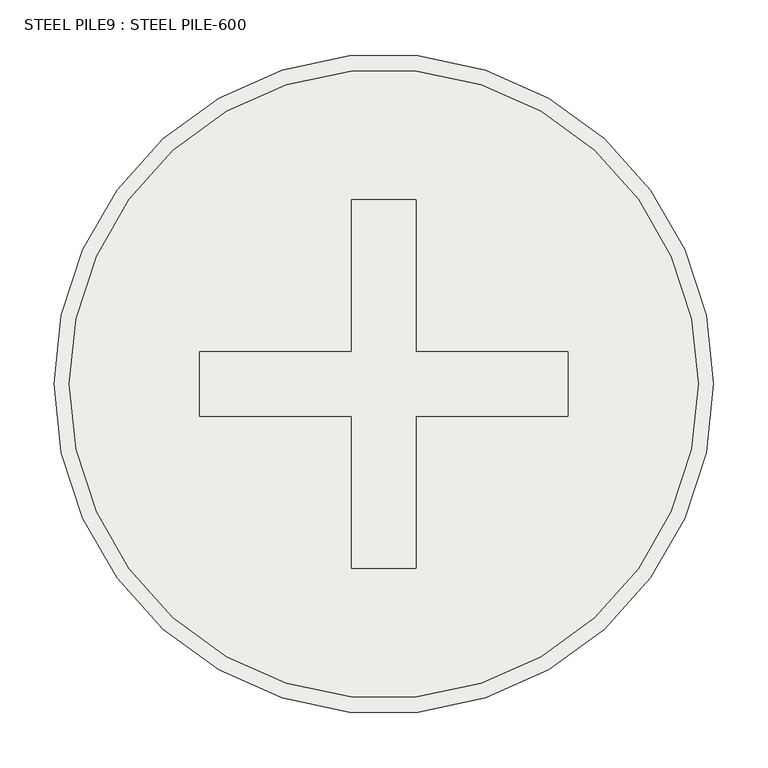
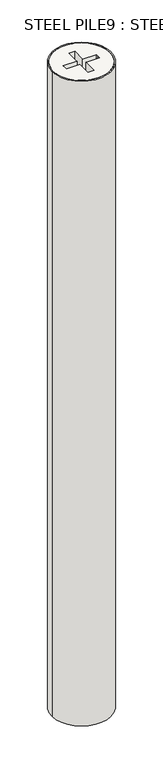
"""IFC4 building model written with IfcOpenShell, lengths in millimetres: slab geometry, STEEL PILE9 : STEEL PILE-600."""

from ifc_helpers import new_model, si_unit, point, frame, frame_2d, origin, place, context, project, spatial, circle_curve, trimmed, segment, composite_curve, outline, extrude, source, transform, mapped, element, save
from ifc_brep_helpers import plane_surface, cylinder_surface, advanced_brep


def steel_pile9_steel_pile_600_482db376(model_context):
    return source(origin(), model_context, "Body", "SolidModel", [
        advanced_brep(
        [(5709.5, 19499.5208589, 150.0), (6290.5, 19499.5208589, 150.0), (5970.0, 19469.5208589, 150.0), (5830.0, 19469.5208589, 150.0), (5830.0, 19499.5208589, 150.0), (5830.0, 19529.5208589, 150.0), (5970.0, 19529.5208589, 150.0), (5970.0, 19669.5208589, 150.0), (6030.0, 19669.5208589, 150.0), (6030.0, 19529.5208589, 150.0), (6170.0, 19529.5208589, 150.0), (6170.0, 19499.5208589, 150.0), (6170.0, 19469.5208589, 150.0), (6030.0, 19469.5208589, 150.0), (6030.0, 19329.5208589, 150.0), (5970.0, 19329.5208589, 150.0), (5709.5, 19499.5208589, -1850.0), (6290.5, 19499.5208589, -1850.0), (5830.0, 19469.5208589, -160.0), (5970.0, 19469.5208589, -160.0), (5970.0, 19329.5208589, -160.0), (6030.0, 19329.5208589, -160.0), (6030.0, 19469.5208589, -160.0), (6170.0, 19469.5208589, -160.0), (6170.0, 19499.5208589, -160.0), (6170.0, 19529.5208589, -160.0), (6030.0, 19529.5208589, -160.0), (6030.0, 19669.5208589, -160.0), (5970.0, 19669.5208589, -160.0), (5970.0, 19529.5208589, -160.0), (5830.0, 19529.5208589, -160.0), (5830.0, 19499.5208589, -160.0)],
        [
            (0, 1, circle_curve(frame((6000.0, 19499.5208589, 150.0), z_axis=(0.0, 0.0, 1.0), x_axis=(1.0, 0.0, 0.0)), 290.5)),
            (1, 0, circle_curve(frame((6000.0, 19499.5208589, 150.0), z_axis=(0.0, 0.0, 1.0), x_axis=(1.0, 0.0, 0.0)), 290.5)),
            (2, 3),
            (3, 4),
            (4, 5),
            (5, 6),
            (6, 7),
            (7, 8),
            (8, 9),
            (9, 10),
            (10, 11),
            (11, 12),
            (12, 13),
            (13, 14),
            (14, 15),
            (15, 2),
            (16, 17, circle_curve(frame((6000.0, 19499.5208589, -1850.0), z_axis=(0.0, 0.0, -1.0), x_axis=(1.0, 0.0, 0.0)), 290.5)),
            (17, 16, circle_curve(frame((6000.0, 19499.5208589, -1850.0), z_axis=(0.0, 0.0, -1.0), x_axis=(1.0, 0.0, 0.0)), 290.5)),
            (0, 16),
            (17, 1),
            (18, 19),
            (19, 20),
            (20, 21),
            (21, 22),
            (22, 23),
            (23, 24),
            (24, 25),
            (25, 26),
            (26, 27),
            (27, 28),
            (28, 29),
            (29, 30),
            (30, 31),
            (31, 18),
            (18, 3),
            (2, 19),
            (15, 20),
            (14, 21),
            (13, 22),
            (12, 23),
            (11, 24),
            (10, 25),
            (9, 26),
            (8, 27),
            (7, 28),
            (6, 29),
            (5, 30),
            (4, 31),
        ],
        [
            plane_surface(frame((6290.5, 19499.5208589, 150.0), z_axis=(0.0, 0.0, 1.0), x_axis=(0.0, 1.0, 0.0))),
            plane_surface(frame((6290.5, 19499.5208589, -1850.0), z_axis=(0.0, 0.0, -1.0), x_axis=(0.0, -1.0, 0.0))),
            cylinder_surface(frame((6000.0, 19499.5208589, -1850.0), z_axis=(0.0, 0.0, 1.0), x_axis=(1.0, 0.0, 0.0)), 290.5),
            plane_surface(frame((5830.0, 19469.5208589, -160.0), z_axis=(0.0, 0.0, 1.0), x_axis=(-1.0, 0.0, 0.0))),
            plane_surface(frame((5830.0, 19469.5208589, 160.0), z_axis=(0.0, 1.0, 0.0), x_axis=(0.0, 0.0, -1.0))),
            plane_surface(frame((5970.0, 19469.5208589, 160.0), z_axis=(1.0, 0.0, 0.0), x_axis=(0.0, 0.0, -1.0))),
            plane_surface(frame((5970.0, 19329.5208589, 160.0), z_axis=(0.0, 1.0, 0.0), x_axis=(0.0, 0.0, -1.0))),
            plane_surface(frame((6030.0, 19329.5208589, 160.0), z_axis=(-1.0, 0.0, 0.0), x_axis=(0.0, 0.0, -1.0))),
            plane_surface(frame((6030.0, 19469.5208589, 160.0), z_axis=(0.0, 1.0, 0.0), x_axis=(0.0, 0.0, -1.0))),
            plane_surface(frame((6170.0, 19469.5208589, 160.0), z_axis=(-1.0, 0.0, 0.0), x_axis=(0.0, 0.0, -1.0))),
            plane_surface(frame((6170.0, 19499.5208589, 160.0), z_axis=(-1.0, 0.0, 0.0), x_axis=(0.0, 0.0, -1.0))),
            plane_surface(frame((6170.0, 19529.5208589, 160.0), z_axis=(0.0, -1.0, 0.0), x_axis=(0.0, 0.0, -1.0))),
            plane_surface(frame((6030.0, 19529.5208589, 160.0), z_axis=(-1.0, 0.0, 0.0), x_axis=(0.0, 0.0, -1.0))),
            plane_surface(frame((6030.0, 19669.5208589, 160.0), z_axis=(0.0, -1.0, 0.0), x_axis=(0.0, 0.0, -1.0))),
            plane_surface(frame((5970.0, 19669.5208589, 160.0), z_axis=(1.0, 0.0, 0.0), x_axis=(0.0, 0.0, -1.0))),
            plane_surface(frame((5970.0, 19529.5208589, 160.0), z_axis=(0.0, -1.0, 0.0), x_axis=(0.0, 0.0, -1.0))),
            plane_surface(frame((5830.0, 19529.5208589, 160.0), z_axis=(1.0, 0.0, 0.0), x_axis=(0.0, 0.0, -1.0))),
            plane_surface(frame((5830.0, 19499.5208589, 160.0), z_axis=(1.0, 0.0, 0.0), x_axis=(0.0, 0.0, -1.0))),
        ],
        [
            (0, [[1, 2], [3, 4, 5, 6, 7, 8, 9, 10, 11, 12, 13, 14, 15, 16]]),
            (1, [[17, 18]]),
            (2, [[-1, 19, -18, 20]]),
            (2, [[-2, -20, -17, -19]]),
            (3, [[21, 22, 23, 24, 25, 26, 27, 28, 29, 30, 31, 32, 33, 34]]),
            (4, [[-21, 35, -3, 36]]),
            (5, [[-22, -36, -16, 37]]),
            (6, [[-23, -37, -15, 38]]),
            (7, [[-24, -38, -14, 39]]),
            (8, [[-25, -39, -13, 40]]),
            (9, [[-26, -40, -12, 41]]),
            (10, [[-27, -41, -11, 42]]),
            (11, [[-28, -42, -10, 43]]),
            (12, [[-29, -43, -9, 44]]),
            (13, [[-30, -44, -8, 45]]),
            (14, [[-31, -45, -7, 46]]),
            (15, [[-32, -46, -6, 47]]),
            (16, [[-33, -47, -5, 48]]),
            (17, [[-34, -48, -4, -35]]),
        ],
    ),
        extrude(outline(composite_curve([segment(trimmed(circle_curve(frame_2d((6000.0, 19499.5208589)), 304.5), [point((5695.5, 19499.5208589))], [point((6304.5, 19499.5208589))], False, "CARTESIAN"), True, "CONTINUOUS"), segment(trimmed(circle_curve(frame_2d((6000.0, 19499.5208589)), 304.5), [point((6304.5, 19499.5208589))], [point((5695.5, 19499.5208589))], False, "CARTESIAN"), True, "CONTINUOUS")], self_intersect=False), holes=[composite_curve([segment(trimmed(circle_curve(frame_2d((6000.0, 19499.5208589)), 290.5), [point((5709.5, 19499.5208589))], [point((6290.5, 19499.5208589))], True, "CARTESIAN"), True, "CONTINUOUS"), segment(trimmed(circle_curve(frame_2d((6000.0, 19499.5208589)), 290.5), [point((6290.5, 19499.5208589))], [point((5709.5, 19499.5208589))], True, "CARTESIAN"), True, "CONTINUOUS")], self_intersect=False)]), frame((0.0, 0.0, -6850.0), z_axis=(0.0, 0.0, 1.0), x_axis=(1.0, 0.0, 0.0)), (0.0, 0.0, 1.0), 7000.0),
    ])


if __name__ == "__main__":
    model = new_model("IFC4")
    model_context = context("Model", 3, world=origin())
    ifc_project = project(units=[si_unit("LENGTHUNIT", "METRE", prefix="MILLI")], contexts=[model_context])
    site = spatial("IfcSite", under=ifc_project)
    building = spatial("IfcBuilding", under=site)
    placement = place(None, origin())
    steel_pile9_steel_pile_600_shape = steel_pile9_steel_pile_600_482db376(model_context)
    element("IfcSlab", 1, ObjectType="STEEL PILE9 : STEEL PILE-600", at=placement, inside=building, context=model_context, shape_type="MappedRepresentation", body=[
        mapped(steel_pile9_steel_pile_600_shape, transform((0.0, 0.0, 0.0), x_axis=(1.0, 0.0, 0.0), y_axis=(0.0, 1.0, 0.0), z_axis=(0.0, 0.0, 1.0))),
    ])
    save(model, "model.ifc")
